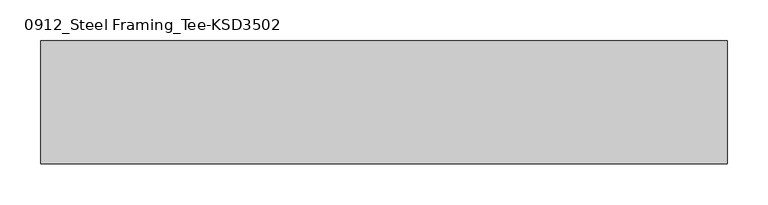
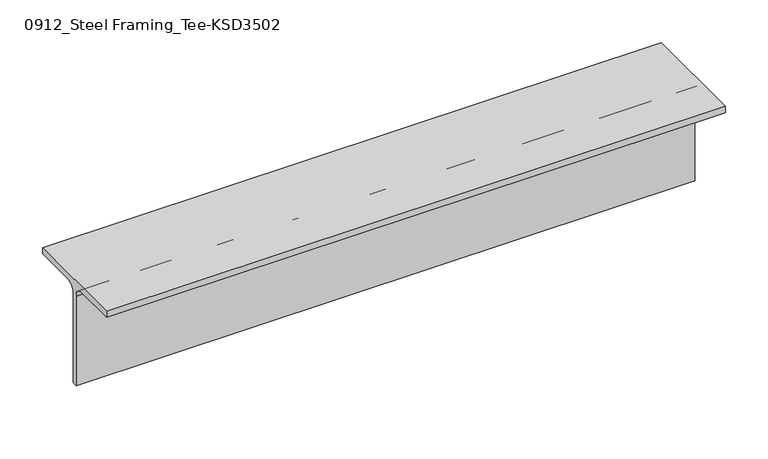
"""IFC4 building model written with IfcOpenShell, lengths in millimetres: member geometry, 0912_Steel Framing_Tee-KSD3502 : H_SB_ASB_CT-150x150x6.5x9."""

import ifcopenshell
import ifcopenshell.guid

model = None  # the IFC model being written
_history = None  # IfcOwnerHistory: only IFC2X3 demands one
_inside = {}  # id of a spatial element -> (the spatial element, [elements in it])
_under = {}  # id of a project, library or spatial element -> (it, [spatial elements below it])
_declared = {}  # id of a project -> (the project, [libraries it declares])
_typed = {}  # id of a type object -> (the type object, [elements of that type])
_made_of = {}  # id of a material, layer set ... -> (it, [elements and type objects made of it])


def new_model(schema):
    """Start an empty IFC model of exactly this schema.

    Asked for "IFC4X3", IfcOpenShell would pick the latest addendum, in which some entities
    have other attributes; the version numbers below select the first issue.
    IFC2X3 requires an IfcOwnerHistory on every rooted entity: one is made here for all.
    """
    global model, _history
    if schema == "IFC4X3":
        model = ifcopenshell.file(schema_version=(4, 3, 0, 0))
    else:
        model = ifcopenshell.file(schema=schema)
    _inside.clear()
    _under.clear()
    _declared.clear()
    _typed.clear()
    _made_of.clear()
    _history = None
    if model.schema == "IFC2X3":
        org = make("IfcOrganization", Name="unknown")
        user = make(
            "IfcPersonAndOrganization",
            ThePerson=make("IfcPerson", FamilyName="unknown"),
            TheOrganization=org,
        )
        app = make(
            "IfcApplication",
            ApplicationDeveloper=org,
            Version="unknown",
            ApplicationFullName="unknown",
            ApplicationIdentifier="unknown",
        )
        _history = make(
            "IfcOwnerHistory",
            OwningUser=user,
            OwningApplication=app,
            ChangeAction="ADDED",
            CreationDate=0,
        )
    return model


def make(cls, **values):
    """One entity of the class cls with the attributes given. An attribute that is None is left unset."""
    return model.create_entity(
        cls, **{name: value for name, value in values.items() if value is not None}
    )


def rooted(cls, **values):
    """An entity with a GlobalId (a new one), such as an element, a storey or a relation."""
    return make(cls, GlobalId=ifcopenshell.guid.new(), OwnerHistory=_history, **values)


def si_unit(unit_type, name, prefix=None):
    """IfcSIUnit, for example si_unit("LENGTHUNIT", "METRE", prefix="MILLI")."""
    return make("IfcSIUnit", UnitType=unit_type, Prefix=prefix, Name=name)


def assignment(units):
    """IfcUnitAssignment: the units of a project."""
    return None if units is None else make("IfcUnitAssignment", Units=units)


def point(xyz):
    """IfcCartesianPoint."""
    return None if xyz is None else make("IfcCartesianPoint", Coordinates=xyz)


def direction(xyz):
    """IfcDirection."""
    return None if xyz is None else make("IfcDirection", DirectionRatios=xyz)


def frame(location, z_axis=None, x_axis=None):
    """IfcAxis2Placement3D, a coordinate frame: its origin and axes. An axis left out is left unset."""
    return make(
        "IfcAxis2Placement3D",
        Location=point(location),
        Axis=direction(z_axis),
        RefDirection=direction(x_axis),
    )


def frame_2d(location, x_axis=None):
    """IfcAxis2Placement2D, a coordinate frame in the plane: its origin and x axis."""
    return make(
        "IfcAxis2Placement2D", Location=point(location), RefDirection=direction(x_axis)
    )


def origin():
    """The frame at (0, 0, 0) with its axes left unset."""
    return frame((0.0, 0.0, 0.0))


def place(relative_to, where):
    """IfcLocalPlacement: puts the frame where relative to a parent placement (None: the world)."""
    return make(
        "IfcLocalPlacement", PlacementRelTo=relative_to, RelativePlacement=where
    )


def context(
    kind, dimensions, precision=None, world=None, true_north=None, identifier=None
):
    """IfcGeometricRepresentationContext, for example the 3D "Model" context."""
    return make(
        "IfcGeometricRepresentationContext",
        ContextIdentifier=identifier,
        ContextType=kind,
        CoordinateSpaceDimension=dimensions,
        Precision=precision,
        WorldCoordinateSystem=world,
        TrueNorth=true_north,
    )


def project(units=None, contexts=None):
    """IfcProject with its units and contexts."""
    return rooted(
        "IfcProject",
        Name="project",
        RepresentationContexts=contexts,
        UnitsInContext=assignment(units),
    )


def spatial(cls, under=None, at=None, **own):
    """A site, building, storey or space (cls), placed at a placement, below another one or the project."""
    s = rooted(cls, ObjectPlacement=at, **own)
    if under is not None:
        _under.setdefault(under.id(), (under, []))[1].append(s)
    return s


def polyline(points):
    """IfcPolyline through the points."""
    return make("IfcPolyline", Points=[point(p) for p in points])


def circle_curve(where, radius):
    """IfcCircle in the frame where."""
    return make("IfcCircle", Position=where, Radius=radius)


def trimmed(basis, trim1, trim2, sense, master):
    """IfcTrimmedCurve: the piece of a basis curve between two trims."""
    return make(
        "IfcTrimmedCurve",
        BasisCurve=basis,
        Trim1=trim1,
        Trim2=trim2,
        SenseAgreement=sense,
        MasterRepresentation=master,
    )


def segment(curve, same_sense, transition):
    """IfcCompositeCurveSegment."""
    return make(
        "IfcCompositeCurveSegment",
        Transition=transition,
        SameSense=same_sense,
        ParentCurve=curve,
    )


def composite_curve(segments, self_intersect=None):
    """IfcCompositeCurve: segments joined end to end."""
    return make("IfcCompositeCurve", Segments=segments, SelfIntersect=self_intersect)


def outline(outer, holes=None, kind="AREA"):
    """IfcArbitraryClosedProfileDef: a profile drawn as a closed curve; with holes, ...WithVoids."""
    if holes is None:
        return make("IfcArbitraryClosedProfileDef", ProfileType=kind, OuterCurve=outer)
    return make(
        "IfcArbitraryProfileDefWithVoids",
        ProfileType=kind,
        OuterCurve=outer,
        InnerCurves=holes,
    )


def extrude(swept, where, along, depth):
    """IfcExtrudedAreaSolid: the profile swept, set in the frame where, extruded along a direction by depth."""
    return make(
        "IfcExtrudedAreaSolid",
        SweptArea=swept,
        Position=where,
        ExtrudedDirection=direction(along),
        Depth=depth,
    )


def shape(context_of_items, identifier, shape_type, items):
    """IfcShapeRepresentation: the items that make up one representation, for example the "Body"."""
    return make(
        "IfcShapeRepresentation",
        ContextOfItems=context_of_items,
        RepresentationIdentifier=identifier,
        RepresentationType=shape_type,
        Items=items,
    )


def source(mapping_origin, context_of_items, identifier, shape_type, items):
    """IfcRepresentationMap: a shape defined once, which mapped items show again and again."""
    return make(
        "IfcRepresentationMap",
        MappingOrigin=mapping_origin,
        MappedRepresentation=shape(context_of_items, identifier, shape_type, items),
    )


def transform(
    local_origin,
    x_axis=None,
    y_axis=None,
    z_axis=None,
    scale=None,
    scale2=None,
    scale3=None,
    uniform=True,
):
    """IfcCartesianTransformationOperator3D, or its non-uniform kind. x_axis, y_axis, z_axis: its Axis1, 2, 3."""
    if uniform:
        return make(
            "IfcCartesianTransformationOperator3D",
            Axis1=direction(x_axis),
            Axis2=direction(y_axis),
            LocalOrigin=point(local_origin),
            Scale=scale,
            Axis3=direction(z_axis),
        )
    return make(
        "IfcCartesianTransformationOperator3DnonUniform",
        Axis1=direction(x_axis),
        Axis2=direction(y_axis),
        LocalOrigin=point(local_origin),
        Scale=scale,
        Axis3=direction(z_axis),
        Scale2=scale2,
        Scale3=scale3,
    )


def mapped(mapping_source, mapping_target):
    """IfcMappedItem: shows the shape of a source again, moved by a transform."""
    return make(
        "IfcMappedItem", MappingSource=mapping_source, MappingTarget=mapping_target
    )


def made_of(thing, what):
    """Note that an element or type object is made of a material, layer set ...; save() writes the relation."""
    if what is not None:
        _made_of.setdefault(what.id(), (what, []))[1].append(thing)
    return thing


def element(
    cls,
    number,
    at=None,
    inside=None,
    cuts=None,
    type_object=None,
    material=None,
    context=None,
    identifier="Body",
    shape_type=None,
    held_by="IfcProductDefinitionShape",
    body=None,
    shapes=None,
    **own,
):
    """One element of the class cls, such as IfcWall. Its Tag is "e" and its number.

    at: its placement. inside: the storey or other place that contains it. cuts: it is an
    opening in that element (IfcRelVoidsElement). A single representation is given by context,
    identifier, shape_type and body (its items); several are given by shapes. held_by: the class
    of the entity that holds the representations. save() writes the other relations.
    """
    e = rooted(cls, Tag="e%d" % number, ObjectPlacement=at, **own)
    if body is not None:
        shapes = [shape(context, identifier, shape_type, body)]
    if shapes is not None:
        e.Representation = make(held_by, Representations=shapes)
    if inside is not None:
        _inside.setdefault(inside.id(), (inside, []))[1].append(e)
    if cuts is not None:
        rooted(
            "IfcRelVoidsElement", RelatingBuildingElement=cuts, RelatedOpeningElement=e
        )
    if type_object is not None:
        _typed.setdefault(type_object.id(), (type_object, []))[1].append(e)
    return made_of(e, material)


def aggregate(whole, parts):
    """IfcRelAggregates: a whole, such as a stair, and the parts it consists of."""
    return rooted("IfcRelAggregates", RelatingObject=whole, RelatedObjects=parts)


def save(model, path):
    """Write the relations noted so far, then the file.

    IfcRelAggregates (storeys below a building ...), IfcRelContainedInSpatialStructure (elements
    in a storey), IfcRelDefinesByType, IfcRelAssociatesMaterial and IfcRelDeclares: one each for
    every whole, place, type object, material and project.
    """
    for whole, parts in _under.values():
        aggregate(whole, parts)
    for where, things in _inside.values():
        rooted(
            "IfcRelContainedInSpatialStructure",
            RelatedElements=things,
            RelatingStructure=where,
        )
    for kind, things in _typed.values():
        rooted("IfcRelDefinesByType", RelatedObjects=things, RelatingType=kind)
    for what, things in _made_of.values():
        rooted("IfcRelAssociatesMaterial", RelatedObjects=things, RelatingMaterial=what)
    for by, libraries in _declared.values():
        rooted("IfcRelDeclares", RelatingContext=by, RelatedDefinitions=libraries)
    model.write(path)


def member_0912_steel_framing_tee_ksd3502_d71e7596(model_context):
    return source(origin(), model_context, "Body", "SweptSolid", [
        extrude(outline(composite_curve([segment(polyline([(-75.0, 75.0), (75.0, 75.0), (75.0, 66.0), (16.25, 66.0)]), True, "CONTINUOUS"), segment(trimmed(circle_curve(frame_2d((16.25, 53.0)), 13.0), [point((16.25, 66.0))], [point((3.25, 53.0))], True, "CARTESIAN"), True, "CONTINUOUS"), segment(polyline([(3.25, 53.0), (3.25, -75.0), (-3.25, -75.0), (-3.25, 53.0)]), True, "CONTINUOUS"), segment(trimmed(circle_curve(frame_2d((-16.25, 53.0)), 13.0), [point((-3.25, 53.0))], [point((-16.25, 66.0))], True, "CARTESIAN"), True, "CONTINUOUS"), segment(polyline([(-16.25, 66.0), (-75.0, 66.0), (-75.0, 75.0)]), True, "CONTINUOUS")], self_intersect=False)), frame((-337.3, 0.0, 0.0), z_axis=(1.0, 0.0, 0.0), x_axis=(0.0, 1.0, 0.0)), (0.0, 0.0, 1.0), 837.3),
    ])


if __name__ == "__main__":
    model = new_model("IFC4")
    model_context = context("Model", 3, world=origin())
    ifc_project = project(units=[si_unit("LENGTHUNIT", "METRE", prefix="MILLI")], contexts=[model_context])
    site = spatial("IfcSite", under=ifc_project)
    building = spatial("IfcBuilding", under=site)
    placement = place(None, origin())
    member_0912_steel_framing_tee_ksd3502_shape = member_0912_steel_framing_tee_ksd3502_d71e7596(model_context)
    element("IfcMember", 1, ObjectType="0912_Steel Framing_Tee-KSD3502 : H_SB_ASB_CT-150x150x6.5x9", at=placement, inside=building, context=model_context, shape_type="MappedRepresentation", body=[
        mapped(member_0912_steel_framing_tee_ksd3502_shape, transform((0.0, 0.0, 0.0), x_axis=(1.0, 0.0, 0.0), y_axis=(0.0, 1.0, 0.0), z_axis=(0.0, 0.0, 1.0))),
    ])
    save(model, "model.ifc")

# Revit data of these elements
# Type "0912_Steel Framing_Tee-KSD3502 : H_SB_ASB_CT-150x150x6.5x9"
#   H_WM Code_1 = "S01AA003-00001 | Main Steel Structure Fabrication Work | Shelter/Building | Light Steel - Standard (30KG/M>Weight) | Material: (   )"
#   H_WM Code_2 = "S03AA029-00001 | Main Steel Structure Erection Work | Shelter/Building | Light Steel (30KG/M>Weight) | Material: (   )"
#   H_WM Code_3 = "S01AA010-00001 | Main Steel Structure Fabrication Work | Shelter/Building | Steel Painting/Coating | for Non-Fireproofed Steel Surface, Surface Preparation, Primer, Second & Final Coat | Material: (   )"
#   H_Q'ty Cal Type Tag = "SB-Q2"
#   Width = 15.0 cm
#   Web Thickness = 0.65 cm
#   Web Fillet = 1.3 cm
#   Section Area = 23.39 cm²
#   Perimeter = 0.60 m²/m
#   Nominal Weight = 18.40 kgf/m
#   Height = 15.0 cm
#   Flange Thickness = 0.9 cm
#   Centroid Vertical = 7.5 cm
#   Centroid Horizontal = 7.5 cm
#   Length [instance default] = 1.5000 m
#   Structural Material [instance default] = Steel, 45-345
#   Warping Constant = (empty or 0)
#   Torsional Moment of Inertia = 0
#   Section Name Key = ""
#   Plastic Modulus weak axis = 0
#   Plastic Modulus strong axis = 0
#   Moment of Inertia weak axis = 0
#   Moment of Inertia strong axis = 0
#   Elastic Modulus weak axis = 0
#   Elastic Modulus strong axis = 0
#   Bolt Spacing = 0
#   Assembly Code = ""
# Element 1 (IfcMember, "0912_Steel Framing_Tee-KSD3502 : H_SB_ASB_CT-150x150x6.5x9")
#   Structural Material = none
# Materials
#   "Steel, 45-345": class "Metal", colour RGB 189 187 185, transparency 0, Description = "Steel 345 MPa", Cost = 0
